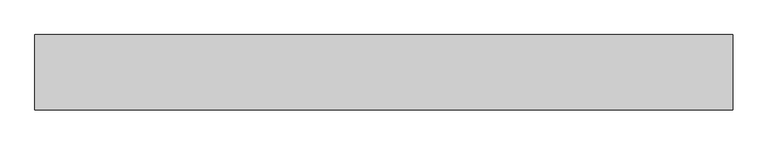
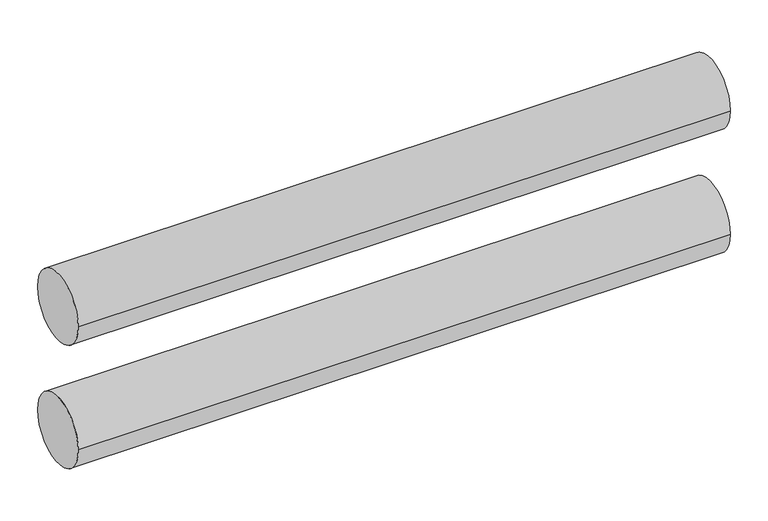
"""IFC4 building model written with IfcOpenShell, lengths in millimetres: proxy geometry, Газпремиум_Регистр : РГТ-1-108х3-1м-2."""

from ifc_helpers import new_model, si_unit, point, frame, frame_2d, origin, place, context, project, spatial, circle_curve, trimmed, segment, composite_curve, outline, extrude, source, transform, mapped, element, save


def mechanical_equipment_34ec048b(model_context):
    return source(origin(), model_context, "Body", "SweptSolid", [
        extrude(outline(composite_curve([segment(trimmed(circle_curve(frame_2d((0.0, 254.0)), 54.0), [point((-54.0, 254.0))], [point((54.0, 254.0))], False, "CARTESIAN"), True, "CONTINUOUS"), segment(trimmed(circle_curve(frame_2d((0.0, 254.0)), 54.0), [point((54.0, 254.0))], [point((-54.0, 254.0))], False, "CARTESIAN"), True, "CONTINUOUS")], self_intersect=False)), frame((315.8280793, 0.0, 0.0), z_axis=(1.0, 0.0, 0.0), x_axis=(0.0, 1.0, 0.0)), (0.0, 0.0, 1.0), 1000.0),
        extrude(outline(composite_curve([segment(trimmed(circle_curve(frame_2d((0.0, 54.0)), 54.0), [point((-54.0, 54.0))], [point((54.0, 54.0))], False, "CARTESIAN"), True, "CONTINUOUS"), segment(trimmed(circle_curve(frame_2d((0.0, 54.0)), 54.0), [point((54.0, 54.0))], [point((-54.0, 54.0))], False, "CARTESIAN"), True, "CONTINUOUS")], self_intersect=False)), frame((315.8280793, 0.0, 0.0), z_axis=(1.0, 0.0, 0.0), x_axis=(0.0, 1.0, 0.0)), (0.0, 0.0, 1.0), 1000.0),
    ])


if __name__ == "__main__":
    model = new_model("IFC4")
    model_context = context("Model", 3, world=origin())
    ifc_project = project(units=[si_unit("LENGTHUNIT", "METRE", prefix="MILLI")], contexts=[model_context])
    site = spatial("IfcSite", under=ifc_project)
    building = spatial("IfcBuilding", under=site)
    placement = place(None, origin())
    mechanical_equipment_shape = mechanical_equipment_34ec048b(model_context)
    element("IfcBuildingElementProxy", 1, Name="Газпремиум_Регистр : РГТ-1-108х3-1м-2", ObjectType="Газпремиум_Регистр : РГТ-1-108х3-1м-2", at=placement, inside=building, context=model_context, shape_type="MappedRepresentation", body=[
        mapped(mechanical_equipment_shape, transform((0.0, 0.0, 0.0), x_axis=(1.0, 0.0, 0.0), y_axis=(0.0, 1.0, 0.0), z_axis=(0.0, 0.0, 1.0))),
    ])
    save(model, "model.ifc")

# Revit data of these elements
# Type "Газпремиум_Регистр : РГТ-1-108х3-1м-2"
#   ADSK_Позиция = "385"
#   ADSK_Наименование = "Регистр однорядный из четырех гладких труб 108х3 длиной 2 м, в комплекте с опорами и экраном"
#   ADSK_Марка = "РГТ-1-108х3-2м-2-ОП-О ТУ 4936-001-69441315-11"
#   ADSK_Код изделия = ""
#   ADSK_Завод-изготовитель = "ООО ПКП \"ГазПремиум\", Россия, г.Саратов, ИНН 6452951387, кпп 645201001, gaz-premium@mail.ru"
#   ADSK_Единица измерения = "шт."
#   Расстояние между рядами = 200 mm
#   Радиус.регистра = 54 mm
#   Отступ.труб.подкл.от.осевой = 32.719 mm
#   Длина регистра = 1000 mm
#   Диаметр.труб.подкл. = 32 mm
#   Диаметр регистра = 108 mm
#   Высота = 200 mm
#   ADSK_Масса = 36.77
#   ADSK_Количество = 1
#   Число рядов = 2
#   Соед.трубы = Грунтовка.красная
#   Регистр = Грунтовка.красная
#   Поддерж.арматура = Грунтовка.серая
#   Default Elevation = 0
# Element 1 (IfcBuildingElementProxy, "Газпремиум_Регистр : РГТ-1-108х3-1м-2")
#   Materials on its faces: "Грунтовка.красная"
# Materials
#   "Грунтовка.красная": class "Разное", colour RGB 255 0 0, transparency 0
#   "Грунтовка.серая": class "Разное", colour RGB 187 181 179, transparency 0
